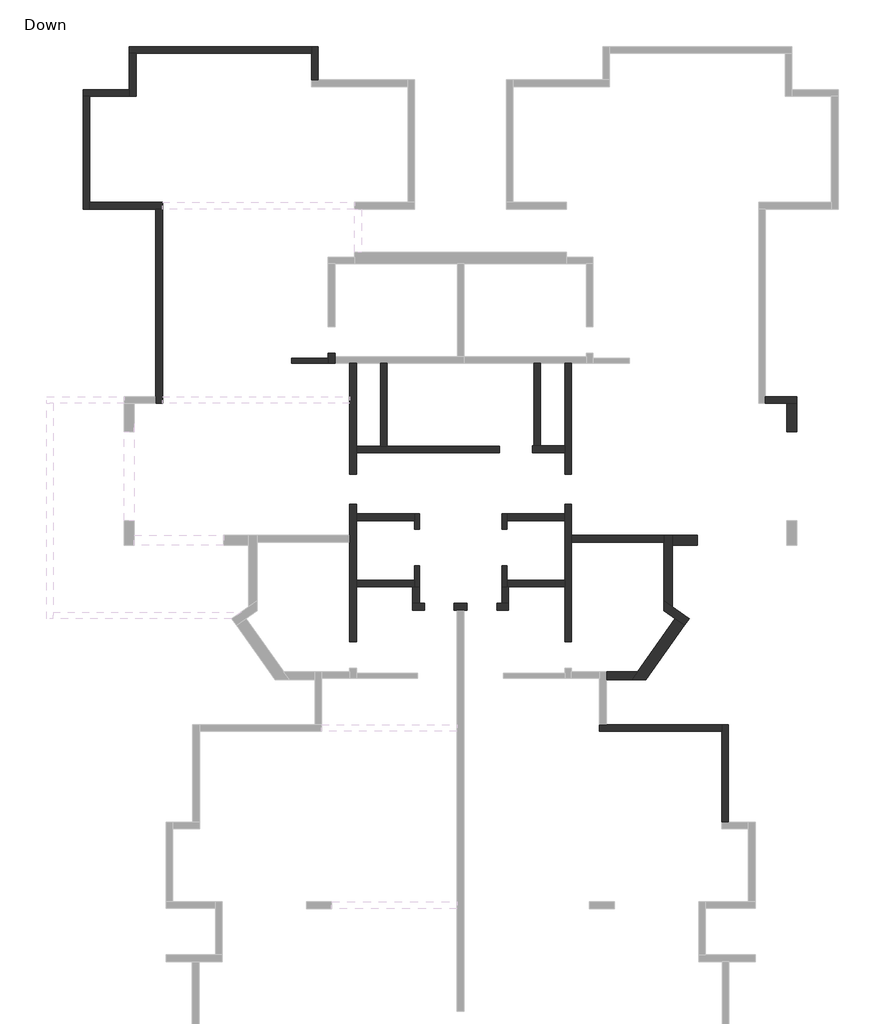
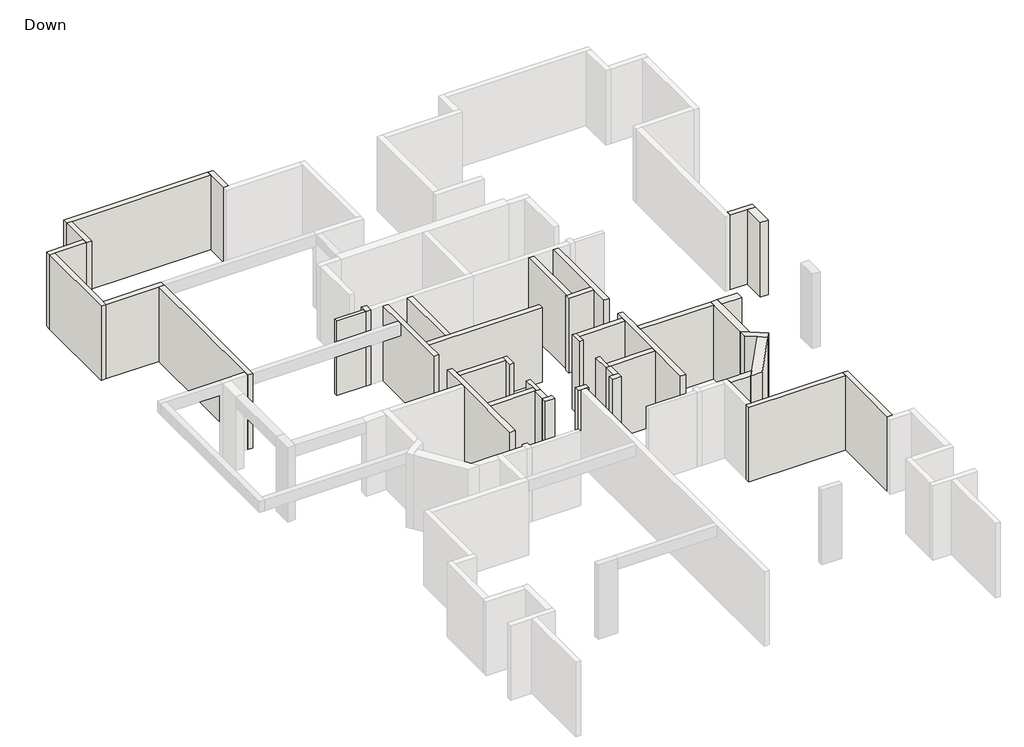
# One storey, part 2 of 3: 40 walls.
"""IFC4 building model written with IfcOpenShell, lengths in millimetres."""

from ifc_helpers import new_model, si_unit, origin, origin_with_axes, place, context, project, spatial, polyline, outline, extrude, faceted_brep, element, save

model = new_model("IFC4")

# Units and contexts
model_context = context("Model", 3, world=origin())
ifc_project = project(units=[si_unit("LENGTHUNIT", "METRE", prefix="MILLI")], contexts=[model_context])

# Site, building, storey
site = spatial("IfcSite", under=ifc_project)
building = spatial("IfcBuilding", under=site)
storey = spatial("IfcBuildingStorey", under=building, Name="Down", Elevation=0.0)

# Walls
placement = place(None, origin())
element("IfcWall", 1, ObjectType="15", at=placement, inside=storey, context=model_context, shape_type="Brep", body=[
    faceted_brep([(27.8998864, 1207.3259107, 0.0), (-1073.0934911, 1207.3259107, 0.0), (-1073.0934911, 1207.3259107, 2800.0), (-1073.0934911, 1207.3259107, 3000.0), (27.8998864, 1207.3259107, 3000.0), (27.8998864, 1207.3259107, 2800.0), (27.8998864, 1057.3259107, 0.0), (27.8998864, 1057.3259107, 3000.0), (-1073.0934911, 1057.3259107, 3000.0), (-1073.0934911, 1057.3259107, 2800.0), (-1073.0934911, 1057.3259107, 0.0)], [[[0, 1, 2, 3, 4, 5]], [[6, 7, 8, 9, 10]], [[1, 0, 6, 10]], [[3, 2, 1, 10, 9, 8]], [[4, 3, 8, 7]], [[0, 5, 4, 7, 6]]]),
])
element("IfcWall", 2, ObjectType="15", at=placement, inside=storey, context=model_context, shape_type="Brep", body=[
    faceted_brep([(2777.2376347, -3950.6211091, 0.0), (2777.2376347, -3491.349586, 0.0), (2777.2376347, -3491.349586, 2800.0), (2777.2376347, -3491.349586, 3000.0), (2777.2376347, -3950.6211091, 3000.0), (2777.2376347, -3950.6211091, 2800.0), (2627.2376347, -3950.6211091, 0.0), (2627.2376347, -3950.6211091, 2800.0), (2627.2376347, -3950.6211091, 3000.0), (2627.2376347, -3691.349586, 3000.0), (2627.2376347, -3491.349586, 3000.0), (2627.2376347, -3491.349586, 0.0), (2627.2376347, -3691.349586, 0.0)], [[[0, 1, 2, 3, 4, 5]], [[6, 7, 8, 9, 10, 11, 12]], [[1, 0, 6, 12, 11]], [[4, 3, 10, 9, 8]], [[0, 5, 4, 8, 7, 6]], [[3, 2, 1, 11, 10]]]),
])
element("IfcWall", 3, ObjectType="15", at=placement, inside=storey, context=model_context, shape_type="Brep", body=[
    faceted_brep([(2777.2376347, -5693.3363409, 0.0), (2777.2376347, -5051.6144866, 0.0), (2777.2376347, -5051.6144866, 2800.0), (2777.2376347, -5051.6144866, 3000.0), (2777.2376347, -5693.3363409, 3000.0), (2627.2376347, -5693.3363409, 0.0), (2627.2376347, -5693.3363409, 3000.0), (2627.2376347, -5493.3363409, 3000.0), (2627.2376347, -5051.6144866, 3000.0), (2627.2376347, -5051.6144866, 2800.0), (2627.2376347, -5051.6144866, 0.0), (2627.2376347, -5493.3363409, 0.0)], [[[0, 1, 2, 3, 4]], [[5, 6, 7, 8, 9, 10, 11]], [[1, 0, 5, 11, 10]], [[3, 2, 1, 10, 9, 8]], [[4, 3, 8, 7, 6]], [[0, 4, 6, 5]]]),
])
element("IfcWall", 4, ObjectType="15", at=placement, inside=storey, context=model_context, shape_type="Brep", body=[
    faceted_brep([(5419.9528665, -3950.6211091, 0.0), (5419.9528665, -3691.349586, 0.0), (5419.9528665, -3491.349586, 0.0), (5419.9528665, -3491.349586, 3000.0), (5419.9528665, -3691.349586, 3000.0), (5419.9528665, -3950.6211091, 3000.0), (5419.9528665, -3950.6211091, 2800.0), (5269.9528665, -3950.6211091, 0.0), (5269.9528665, -3950.6211091, 2800.0), (5269.9528665, -3950.6211091, 3000.0), (5269.9528665, -3491.349586, 3000.0), (5269.9528665, -3491.349586, 2800.0), (5269.9528665, -3491.349586, 0.0)], [[[0, 1, 2, 3, 4, 5, 6]], [[7, 8, 9, 10, 11, 12]], [[2, 1, 0, 7, 12]], [[5, 4, 3, 10, 9]], [[0, 6, 5, 9, 8, 7]], [[3, 2, 12, 11, 10]]]),
])
element("IfcWall", 5, ObjectType="15", at=placement, inside=storey, context=model_context, shape_type="Brep", body=[
    faceted_brep([(5419.9528665, -5693.3363409, 0.0), (5419.9528665, -5493.3363409, 0.0), (5419.9528665, -5051.6144866, 0.0), (5419.9528665, -5051.6144866, 2800.0), (5419.9528665, -5051.6144866, 3000.0), (5419.9528665, -5493.3363409, 3000.0), (5419.9528665, -5693.3363409, 3000.0), (5269.9528665, -5693.3363409, 0.0), (5269.9528665, -5693.3363409, 3000.0), (5269.9528665, -5051.6144866, 3000.0), (5269.9528665, -5051.6144866, 2800.0), (5269.9528665, -5051.6144866, 0.0)], [[[0, 1, 2, 3, 4, 5, 6]], [[7, 8, 9, 10, 11]], [[2, 1, 0, 7, 11]], [[4, 3, 2, 11, 10, 9]], [[6, 5, 4, 9, 8]], [[0, 6, 8, 7]]]),
])
element("IfcWall", 6, ObjectType="20", at=placement, inside=storey, context=model_context, shape_type="Brep", body=[
    faceted_brep([(-275.4113719, 9607.9881624, 0.0), (-275.4113719, 10613.9484273, 0.0), (-275.4113719, 10613.9484273, 3000.0), (-275.4113719, 9607.9881624, 3000.0), (-475.4113719, 9607.9881624, 0.0), (-475.4113719, 9607.9881624, 3000.0), (-475.4113719, 10413.9484273, 3000.0), (-475.4113719, 10613.9484273, 3000.0), (-475.4113719, 10613.9484273, 0.0), (-475.4113719, 10413.9484273, 0.0)], [[[0, 1, 2, 3]], [[4, 5, 6, 7, 8, 9]], [[1, 0, 4, 9, 8]], [[3, 2, 7, 6, 5]], [[0, 3, 5, 4]], [[2, 1, 8, 7]]]),
])
element("IfcWall", 7, ObjectType="20", at=placement, inside=storey, context=model_context, shape_type="Brep", body=[
    faceted_brep([(-475.4113719, 10613.9484273, 0.0), (-5975.4113719, 10613.9484273, 0.0), (-5975.4113719, 10613.9484273, 3000.0), (-475.4113719, 10613.9484273, 3000.0), (-475.4113719, 10413.9484273, 0.0), (-475.4113719, 10413.9484273, 2800.0), (-475.4113719, 10413.9484273, 3000.0), (-5775.4113719, 10413.9484273, 3000.0), (-5975.4113719, 10413.9484273, 3000.0), (-5975.4113719, 10413.9484273, 0.0), (-5775.4113719, 10413.9484273, 0.0)], [[[0, 1, 2, 3]], [[4, 5, 6, 7, 8, 9, 10]], [[1, 0, 4, 10, 9]], [[3, 2, 8, 7, 6]], [[0, 3, 6, 5, 4]], [[2, 1, 9, 8]]]),
])
element("IfcWall", 8, ObjectType="20", at=placement, inside=storey, context=model_context, shape_type="Brep", body=[
    faceted_brep([(-5975.4113719, 10413.9484273, 0.0), (-5975.4113719, 9310.3060432, 0.0), (-5975.4113719, 9110.3060432, 0.0), (-5975.4113719, 9110.3060432, 3000.0), (-5975.4113719, 9310.3060432, 3000.0), (-5975.4113719, 10413.9484273, 3000.0), (-5775.4113719, 10413.9484273, 0.0), (-5775.4113719, 10413.9484273, 2800.0), (-5775.4113719, 10413.9484273, 3000.0), (-5775.4113719, 9110.3060432, 3000.0), (-5775.4113719, 9110.3060432, 2800.0), (-5775.4113719, 9110.3060432, 0.0)], [[[0, 1, 2, 3, 4, 5]], [[6, 7, 8, 9, 10, 11]], [[2, 1, 0, 6, 11]], [[5, 4, 3, 9, 8]], [[0, 5, 8, 7, 6]], [[3, 2, 11, 10, 9]]]),
])
element("IfcWall", 9, ObjectType="20", at=placement, inside=storey, context=model_context, shape_type="Brep", body=[
    faceted_brep([(-5975.4113719, 9310.3060432, 0.0), (-7377.0670011, 9310.3060432, 0.0), (-7377.0670011, 9310.3060432, 3000.0), (-5975.4113719, 9310.3060432, 3000.0), (-5975.4113719, 9110.3060432, 0.0), (-5975.4113719, 9110.3060432, 3000.0), (-7177.0670011, 9110.3060432, 3000.0), (-7377.0670011, 9110.3060432, 3000.0), (-7377.0670011, 9110.3060432, 0.0), (-7177.0670011, 9110.3060432, 0.0)], [[[0, 1, 2, 3]], [[4, 5, 6, 7, 8, 9]], [[1, 0, 4, 9, 8]], [[3, 2, 7, 6, 5]], [[0, 3, 5, 4]], [[2, 1, 8, 7]]]),
])
element("IfcWall", 10, ObjectType="20", at=placement, inside=storey, context=model_context, shape_type="Brep", body=[
    faceted_brep([(-7377.0670011, 9110.3060432, 0.0), (-7377.0670011, 5707.9881624, 0.0), (-7377.0670011, 5707.9881624, 3000.0), (-7377.0670011, 9110.3060432, 3000.0), (-7177.0670011, 9110.3060432, 0.0), (-7177.0670011, 9110.3060432, 2800.0), (-7177.0670011, 9110.3060432, 3000.0), (-7177.0670011, 5907.9881624, 3000.0), (-7177.0670011, 5707.9881624, 3000.0), (-7177.0670011, 5707.9881624, 0.0), (-7177.0670011, 5907.9881624, 0.0)], [[[0, 1, 2, 3]], [[4, 5, 6, 7, 8, 9, 10]], [[1, 0, 4, 10, 9]], [[3, 2, 8, 7, 6]], [[0, 3, 6, 5, 4]], [[2, 1, 9, 8]]]),
])
element("IfcWall", 11, ObjectType="20", at=placement, inside=storey, context=model_context, shape_type="Brep", body=[
    faceted_brep([(-7177.0670011, 5707.9881624, 0.0), (-5177.0670011, 5707.9881624, 0.0), (-4977.0670011, 5707.9881624, 0.0), (-4977.0670011, 5707.9881624, 2550.0), (-4977.0670011, 5707.9881624, 3000.0), (-5177.0670011, 5707.9881624, 3000.0), (-7177.0670011, 5707.9881624, 3000.0), (-7177.0670011, 5907.9881624, 0.0), (-7177.0670011, 5907.9881624, 2800.0), (-7177.0670011, 5907.9881624, 3000.0), (-4977.0670011, 5907.9881624, 3000.0), (-4977.0670011, 5907.9881624, 2550.0), (-4977.0670011, 5907.9881624, 0.0)], [[[0, 1, 2, 3, 4, 5, 6]], [[7, 8, 9, 10, 11, 12]], [[2, 1, 0, 7, 12]], [[6, 5, 4, 10, 9]], [[0, 6, 9, 8, 7]], [[4, 3, 2, 12, 11, 10]]]),
])
element("IfcWall", 12, ObjectType="20", at=placement, inside=storey, context=model_context, shape_type="Brep", body=[
    faceted_brep([(-5177.0670011, 5707.9881624, 0.0), (-5177.0670011, 46.6636591, 0.0), (-5177.0670011, -153.3363409, 0.0), (-5177.0670011, -153.3363409, 3000.0), (-5177.0670011, 46.6636591, 3000.0), (-5177.0670011, 5707.9881624, 3000.0), (-4977.0670011, 5707.9881624, 0.0), (-4977.0670011, 5707.9881624, 2800.0), (-4977.0670011, 5707.9881624, 3000.0), (-4977.0670011, 46.6636591, 3000.0), (-4977.0670011, -153.3363409, 3000.0), (-4977.0670011, -153.3363409, 0.0)], [[[0, 1, 2, 3, 4, 5]], [[6, 7, 8, 9, 10, 11]], [[2, 1, 0, 6, 11]], [[5, 4, 3, 10, 9, 8]], [[0, 5, 8, 7, 6]], [[3, 2, 11, 10]]]),
])
element("IfcWall", 13, ObjectType="20", at=placement, inside=storey, context=model_context, shape_type="Brep", body=[
    faceted_brep([(27.8998864, 1353.021275, 0.0), (27.8998864, 1207.3259107, 0.0), (27.8998864, 1057.3259107, 0.0), (27.8998864, 1057.3259107, 3000.0), (27.8998864, 1207.3259107, 3000.0), (27.8998864, 1353.021275, 3000.0), (27.8998864, 1353.021275, 2800.0), (227.8998864, 1353.021275, 0.0), (227.8998864, 1353.021275, 2800.0), (227.8998864, 1353.021275, 3000.0), (227.8998864, 1257.3259107, 3000.0), (227.8998864, 1057.3259107, 3000.0), (227.8998864, 1057.3259107, 0.0), (227.8998864, 1257.3259107, 0.0)], [[[0, 1, 2, 3, 4, 5, 6]], [[7, 8, 9, 10, 11, 12, 13]], [[2, 1, 0, 7, 13, 12]], [[5, 4, 3, 11, 10, 9]], [[0, 6, 5, 9, 8, 7]], [[3, 2, 12, 11]]]),
])
element("IfcWall", 14, ObjectType="20", at=placement, inside=storey, context=model_context, shape_type="Brep", body=[
    faceted_brep([(675.9131314, 1057.3259107, 0.0), (675.9131314, -2295.9853475, 0.0), (675.9131314, -2295.9853475, 2800.0), (675.9131314, -2295.9853475, 3000.0), (675.9131314, -153.3363409, 3000.0), (675.9131314, 46.6636591, 3000.0), (675.9131314, 1057.3259107, 3000.0), (675.9131314, 1057.3259107, 2800.0), (875.9131314, 1057.3259107, 0.0), (875.9131314, 1057.3259107, 3000.0), (875.9131314, -1441.6807118, 3000.0), (875.9131314, -1641.6807118, 3000.0), (875.9131314, -2295.9853475, 3000.0), (875.9131314, -2295.9853475, 2800.0), (875.9131314, -2295.9853475, 0.0), (875.9131314, -1641.6807118, 0.0), (875.9131314, -1441.6807118, 0.0)], [[[0, 1, 2, 3, 4, 5, 6, 7]], [[8, 9, 10, 11, 12, 13, 14, 15, 16]], [[1, 0, 8, 16, 15, 14]], [[3, 2, 1, 14, 13, 12]], [[6, 5, 4, 3, 12, 11, 10, 9]], [[0, 7, 6, 9, 8]]]),
])
element("IfcWall", 15, ObjectType="20", at=placement, inside=storey, context=model_context, shape_type="Brep", body=[
    faceted_brep([(875.9131314, -1641.6807118, 0.0), (5199.4230652, -1641.6807118, 0.0), (5199.4230652, -1641.6807118, 2800.0), (5199.4230652, -1641.6807118, 3000.0), (875.9131314, -1641.6807118, 3000.0), (875.9131314, -1641.6807118, 2800.0), (875.9131314, -1441.6807118, 0.0), (875.9131314, -1441.6807118, 3000.0), (1608.3634625, -1441.6807118, 3000.0), (1808.3634625, -1441.6807118, 3000.0), (5199.4230652, -1441.6807118, 3000.0), (5199.4230652, -1441.6807118, 2800.0), (5199.4230652, -1441.6807118, 0.0), (1808.3634625, -1441.6807118, 0.0), (1608.3634625, -1441.6807118, 0.0)], [[[0, 1, 2, 3, 4, 5]], [[6, 7, 8, 9, 10, 11, 12, 13, 14]], [[1, 0, 6, 14, 13, 12]], [[3, 2, 1, 12, 11, 10]], [[4, 3, 10, 9, 8, 7]], [[0, 5, 4, 7, 6]]]),
])
element("IfcWall", 16, ObjectType="20", at=placement, inside=storey, context=model_context, shape_type="SweptSolid", body=[
    extrude(outline(polyline([(1808.3634625, 1057.3259107), (1808.3634625, -1441.6807118), (1608.3634625, -1441.6807118), (1608.3634625, 1057.3259107), (1808.3634625, 1057.3259107)])), origin_with_axes(), (0.0, 0.0, 1.0), 3000.0),
])
element("IfcWall", 17, ObjectType="20", at=placement, inside=storey, context=model_context, shape_type="Brep", body=[
    faceted_brep([(675.9131314, -3195.6542217, 0.0), (675.9131314, -4140.6873343, 0.0), (675.9131314, -4340.6873343, 0.0), (675.9131314, -7341.6807118, 0.0), (675.9131314, -7341.6807118, 2800.0), (675.9131314, -7341.6807118, 3000.0), (675.9131314, -4340.6873343, 3000.0), (675.9131314, -4140.6873343, 3000.0), (675.9131314, -3195.6542217, 3000.0), (675.9131314, -3195.6542217, 2800.0), (875.9131314, -3195.6542217, 0.0), (875.9131314, -3195.6542217, 2800.0), (875.9131314, -3195.6542217, 3000.0), (875.9131314, -3491.349586, 3000.0), (875.9131314, -3691.349586, 3000.0), (875.9131314, -5493.3363409, 3000.0), (875.9131314, -5693.3363409, 3000.0), (875.9131314, -7341.6807118, 3000.0), (875.9131314, -7341.6807118, 2800.0), (875.9131314, -7341.6807118, 0.0), (875.9131314, -5693.3363409, 0.0), (875.9131314, -5493.3363409, 0.0), (875.9131314, -3691.349586, 0.0), (875.9131314, -3491.349586, 0.0)], [[[0, 1, 2, 3, 4, 5, 6, 7, 8, 9]], [[10, 11, 12, 13, 14, 15, 16, 17, 18, 19, 20, 21, 22, 23]], [[3, 2, 1, 0, 10, 23, 22, 21, 20, 19]], [[5, 4, 3, 19, 18, 17]], [[8, 7, 6, 5, 17, 16, 15, 14, 13, 12]], [[0, 9, 8, 12, 11, 10]]]),
])
element("IfcWall", 18, ObjectType="20", at=placement, inside=storey, context=model_context, shape_type="Brep", body=[
    faceted_brep([(875.9131314, -5693.3363409, 0.0), (2577.2376347, -5693.3363409, 0.0), (2627.2376347, -5693.3363409, 0.0), (2627.2376347, -5693.3363409, 3000.0), (2577.2376347, -5693.3363409, 3000.0), (875.9131314, -5693.3363409, 3000.0), (875.9131314, -5693.3363409, 2800.0), (875.9131314, -5493.3363409, 0.0), (875.9131314, -5493.3363409, 3000.0), (2627.2376347, -5493.3363409, 3000.0), (2627.2376347, -5493.3363409, 0.0)], [[[0, 1, 2, 3, 4, 5, 6]], [[7, 8, 9, 10]], [[2, 1, 0, 7, 10]], [[5, 4, 3, 9, 8]], [[0, 6, 5, 8, 7]], [[3, 2, 10, 9]]]),
])
element("IfcWall", 19, ObjectType="20", at=placement, inside=storey, context=model_context, shape_type="Brep", body=[
    faceted_brep([(2627.2376347, -3491.349586, 0.0), (875.9131314, -3491.349586, 0.0), (875.9131314, -3491.349586, 2800.0), (875.9131314, -3491.349586, 3000.0), (2627.2376347, -3491.349586, 3000.0), (2627.2376347, -3691.349586, 0.0), (2627.2376347, -3691.349586, 3000.0), (875.9131314, -3691.349586, 3000.0), (875.9131314, -3691.349586, 0.0)], [[[0, 1, 2, 3, 4]], [[5, 6, 7, 8]], [[1, 0, 5, 8]], [[4, 3, 7, 6]], [[0, 4, 6, 5]], [[3, 2, 1, 8, 7]]]),
])
element("IfcWall", 20, ObjectType="20", at=placement, inside=storey, context=model_context, shape_type="Brep", body=[
    faceted_brep([(2577.2376347, -5693.3363409, 0.0), (2577.2376347, -6191.6807118, 0.0), (2577.2376347, -6191.6807118, 3000.0), (2577.2376347, -5693.3363409, 3000.0), (2577.2376347, -5693.3363409, 2800.0), (2777.2376347, -5693.3363409, 0.0), (2777.2376347, -5693.3363409, 3000.0), (2777.2376347, -6191.6807118, 3000.0), (2777.2376347, -6191.6807118, 2800.0), (2777.2376347, -6191.6807118, 0.0), (2627.2376347, -5693.3363409, 0.0), (2627.2376347, -5693.3363409, 3000.0)], [[[0, 1, 2, 3, 4]], [[5, 6, 7, 8, 9]], [[1, 0, 10, 5, 9]], [[3, 2, 7, 6, 11]], [[0, 4, 3, 11, 6, 5, 10]], [[2, 1, 9, 8, 7]]]),
])
element("IfcWall", 21, ObjectType="20", at=placement, inside=storey, context=model_context, shape_type="Brep", body=[
    faceted_brep([(2577.2376347, -6391.6807118, 0.0), (2928.2310122, -6391.6807118, 0.0), (2928.2310122, -6391.6807118, 2800.0), (2928.2310122, -6391.6807118, 3000.0), (2577.2376347, -6391.6807118, 3000.0), (2577.2376347, -6391.6807118, 2800.0), (2577.2376347, -6191.6807118, 0.0), (2577.2376347, -6191.6807118, 3000.0), (2777.2376347, -6191.6807118, 3000.0), (2928.2310122, -6191.6807118, 3000.0), (2928.2310122, -6191.6807118, 2800.0), (2928.2310122, -6191.6807118, 0.0), (2777.2376347, -6191.6807118, 0.0)], [[[0, 1, 2, 3, 4, 5]], [[6, 7, 8, 9, 10, 11, 12]], [[1, 0, 6, 12, 11]], [[3, 2, 1, 11, 10, 9]], [[4, 3, 9, 8, 7]], [[0, 5, 4, 7, 6]]]),
])
element("IfcWall", 22, ObjectType="20", at=placement, inside=storey, context=model_context, shape_type="Brep", body=[
    faceted_brep([(3827.8998864, -6391.6807118, 0.0), (3923.5952506, -6391.6807118, 0.0), (4123.5952506, -6391.6807118, 0.0), (4224.2575022, -6391.6807118, 0.0), (4224.2575022, -6391.6807118, 2800.0), (4224.2575022, -6391.6807118, 3000.0), (4123.5952506, -6391.6807118, 3000.0), (3923.5952506, -6391.6807118, 3000.0), (3827.8998864, -6391.6807118, 3000.0), (3827.8998864, -6391.6807118, 2800.0), (3827.8998864, -6191.6807118, 0.0), (3827.8998864, -6191.6807118, 2800.0), (3827.8998864, -6191.6807118, 3000.0), (4224.2575022, -6191.6807118, 3000.0), (4224.2575022, -6191.6807118, 2800.0), (4224.2575022, -6191.6807118, 0.0)], [[[0, 1, 2, 3, 4, 5, 6, 7, 8, 9]], [[10, 11, 12, 13, 14, 15]], [[3, 2, 1, 0, 10, 15]], [[5, 4, 3, 15, 14, 13]], [[8, 7, 6, 5, 13, 12]], [[0, 9, 8, 12, 11, 10]]]),
])
element("IfcWall", 23, ObjectType="20", at=placement, inside=storey, context=model_context, shape_type="Brep", body=[
    faceted_brep([(13224.2575022, -153.3363409, 0.0), (13875.1499872, -153.3363409, 0.0), (14175.1499872, -153.3363409, 0.0), (14175.1499872, -153.3363409, 2550.0), (14175.1499872, -153.3363409, 3000.0), (13875.1499872, -153.3363409, 3000.0), (13224.2575022, -153.3363409, 3000.0), (13224.2575022, 46.6636591, 0.0), (13224.2575022, 46.6636591, 3000.0), (14175.1499872, 46.6636591, 3000.0), (14175.1499872, 46.6636591, 2550.0), (14175.1499872, 46.6636591, 0.0)], [[[0, 1, 2, 3, 4, 5, 6]], [[7, 8, 9, 10, 11]], [[2, 1, 0, 7, 11]], [[6, 5, 4, 9, 8]], [[0, 6, 8, 7]], [[4, 3, 2, 11, 10, 9]]]),
])
element("IfcWall", 24, ObjectType="20", at=placement, inside=storey, context=model_context, shape_type="Brep", body=[
    faceted_brep([(7169.9528665, 1057.3259107, 0.0), (7169.9528665, -1440.3562085, 0.0), (7169.9528665, -1640.3562085, 0.0), (7169.9528665, -2295.9853475, 0.0), (7169.9528665, -2295.9853475, 2800.0), (7169.9528665, -2295.9853475, 3000.0), (7169.9528665, -1640.3562085, 3000.0), (7169.9528665, -1440.3562085, 3000.0), (7169.9528665, 1057.3259107, 3000.0), (7369.9528665, 1057.3259107, 0.0), (7369.9528665, 1057.3259107, 2800.0), (7369.9528665, 1057.3259107, 3000.0), (7369.9528665, 46.6636591, 3000.0), (7369.9528665, -153.3363409, 3000.0), (7369.9528665, -2295.9853475, 3000.0), (7369.9528665, -2295.9853475, 2800.0), (7369.9528665, -2295.9853475, 0.0)], [[[0, 1, 2, 3, 4, 5, 6, 7, 8]], [[9, 10, 11, 12, 13, 14, 15, 16]], [[3, 2, 1, 0, 9, 16]], [[5, 4, 3, 16, 15, 14]], [[8, 7, 6, 5, 14, 13, 12, 11]], [[0, 8, 11, 10, 9]]]),
])
element("IfcWall", 25, ObjectType="20", at=placement, inside=storey, context=model_context, shape_type="SweptSolid", body=[
    extrude(outline(polyline([(6438.8270387, 1057.3259107), (6438.8270387, -1440.3562085), (6238.8270387, -1440.3562085), (6238.8270387, 1057.3259107), (6438.8270387, 1057.3259107)])), origin_with_axes(), (0.0, 0.0, 1.0), 3000.0),
])
element("IfcWall", 26, ObjectType="20", at=placement, inside=storey, context=model_context, shape_type="Brep", body=[
    faceted_brep([(7169.9528665, -3195.6542217, 0.0), (7169.9528665, -3491.349586, 0.0), (7169.9528665, -3691.349586, 0.0), (7169.9528665, -5493.3363409, 0.0), (7169.9528665, -5693.3363409, 0.0), (7169.9528665, -7341.6807118, 0.0), (7169.9528665, -7341.6807118, 2800.0), (7169.9528665, -7341.6807118, 3000.0), (7169.9528665, -5693.3363409, 3000.0), (7169.9528665, -5493.3363409, 3000.0), (7169.9528665, -3691.349586, 3000.0), (7169.9528665, -3491.349586, 3000.0), (7169.9528665, -3195.6542217, 3000.0), (7169.9528665, -3195.6542217, 2800.0), (7369.9528665, -3195.6542217, 0.0), (7369.9528665, -3195.6542217, 2800.0), (7369.9528665, -3195.6542217, 3000.0), (7369.9528665, -4140.6873343, 3000.0), (7369.9528665, -4340.6873343, 3000.0), (7369.9528665, -7341.6807118, 3000.0), (7369.9528665, -7341.6807118, 2800.0), (7369.9528665, -7341.6807118, 0.0), (7369.9528665, -4340.6873343, 0.0), (7369.9528665, -4140.6873343, 0.0)], [[[0, 1, 2, 3, 4, 5, 6, 7, 8, 9, 10, 11, 12, 13]], [[14, 15, 16, 17, 18, 19, 20, 21, 22, 23]], [[5, 4, 3, 2, 1, 0, 14, 23, 22, 21]], [[7, 6, 5, 21, 20, 19]], [[12, 11, 10, 9, 8, 7, 19, 18, 17, 16]], [[0, 13, 12, 16, 15, 14]]]),
])
element("IfcWall", 27, ObjectType="20", at=placement, inside=storey, context=model_context, shape_type="Brep", body=[
    faceted_brep([(7169.9528665, -5493.3363409, 0.0), (5419.9528665, -5493.3363409, 0.0), (5419.9528665, -5493.3363409, 3000.0), (7169.9528665, -5493.3363409, 3000.0), (7169.9528665, -5693.3363409, 0.0), (7169.9528665, -5693.3363409, 2800.0), (7169.9528665, -5693.3363409, 3000.0), (5469.9528665, -5693.3363409, 3000.0), (5419.9528665, -5693.3363409, 3000.0), (5419.9528665, -5693.3363409, 0.0), (5469.9528665, -5693.3363409, 0.0)], [[[0, 1, 2, 3]], [[4, 5, 6, 7, 8, 9, 10]], [[1, 0, 4, 10, 9]], [[3, 2, 8, 7, 6]], [[0, 3, 6, 5, 4]], [[2, 1, 9, 8]]]),
])
element("IfcWall", 28, ObjectType="20", at=placement, inside=storey, context=model_context, shape_type="Brep", body=[
    faceted_brep([(5419.9528665, -3691.349586, 0.0), (7169.9528665, -3691.349586, 0.0), (7169.9528665, -3691.349586, 3000.0), (5419.9528665, -3691.349586, 3000.0), (5419.9528665, -3491.349586, 0.0), (5419.9528665, -3491.349586, 3000.0), (7169.9528665, -3491.349586, 3000.0), (7169.9528665, -3491.349586, 2800.0), (7169.9528665, -3491.349586, 0.0)], [[[0, 1, 2, 3]], [[4, 5, 6, 7, 8]], [[1, 0, 4, 8]], [[3, 2, 6, 5]], [[0, 3, 5, 4]], [[2, 1, 8, 7, 6]]]),
])
element("IfcWall", 29, ObjectType="20", at=placement, inside=storey, context=model_context, shape_type="Brep", body=[
    faceted_brep([(5269.9528665, -5693.3363409, 0.0), (5269.9528665, -6191.6807118, 0.0), (5269.9528665, -6191.6807118, 2800.0), (5269.9528665, -6191.6807118, 3000.0), (5269.9528665, -5693.3363409, 3000.0), (5469.9528665, -5693.3363409, 0.0), (5469.9528665, -5693.3363409, 2800.0), (5469.9528665, -5693.3363409, 3000.0), (5469.9528665, -6191.6807118, 3000.0), (5469.9528665, -6191.6807118, 0.0), (5419.9528665, -5693.3363409, 0.0), (5419.9528665, -5693.3363409, 3000.0)], [[[0, 1, 2, 3, 4]], [[5, 6, 7, 8, 9]], [[1, 0, 10, 5, 9]], [[4, 3, 8, 7, 11]], [[0, 4, 11, 7, 6, 5, 10]], [[3, 2, 1, 9, 8]]]),
])
element("IfcWall", 30, ObjectType="20", at=placement, inside=storey, context=model_context, shape_type="Brep", body=[
    faceted_brep([(5469.9528665, -6191.6807118, 0.0), (5269.9528665, -6191.6807118, 0.0), (5118.959489, -6191.6807118, 0.0), (5118.959489, -6191.6807118, 2800.0), (5118.959489, -6191.6807118, 3000.0), (5269.9528665, -6191.6807118, 3000.0), (5469.9528665, -6191.6807118, 3000.0), (5469.9528665, -6391.6807118, 0.0), (5469.9528665, -6391.6807118, 2800.0), (5469.9528665, -6391.6807118, 3000.0), (5118.959489, -6391.6807118, 3000.0), (5118.959489, -6391.6807118, 2800.0), (5118.959489, -6391.6807118, 0.0)], [[[0, 1, 2, 3, 4, 5, 6]], [[7, 8, 9, 10, 11, 12]], [[2, 1, 0, 7, 12]], [[4, 3, 2, 12, 11, 10]], [[6, 5, 4, 10, 9]], [[0, 6, 9, 8, 7]]]),
])
element("IfcWall", 31, ObjectType="20", at=placement, inside=storey, context=model_context, shape_type="Brep", body=[
    faceted_brep([(12107.370085, -12796.3164734, 0.0), (12107.370085, -9845.6542217, 0.0), (12107.370085, -9845.6542217, 3000.0), (12107.370085, -12796.3164734, 3000.0), (11907.370085, -12796.3164734, 0.0), (11907.370085, -12796.3164734, 3000.0), (11907.370085, -10045.6542217, 3000.0), (11907.370085, -9845.6542217, 3000.0), (11907.370085, -9845.6542217, 0.0), (11907.370085, -10045.6542217, 0.0)], [[[0, 1, 2, 3]], [[4, 5, 6, 7, 8, 9]], [[1, 0, 4, 9, 8]], [[3, 2, 7, 6, 5]], [[0, 3, 5, 4]], [[2, 1, 8, 7]]]),
])
element("IfcWall", 32, ObjectType="20", at=placement, inside=storey, context=model_context, shape_type="Brep", body=[
    faceted_brep([(11907.370085, -9845.6542217, 0.0), (8420.6151181, -9845.6542217, 0.0), (8220.6151181, -9845.6542217, 0.0), (8220.6151181, -9845.6542217, 2550.0), (8220.6151181, -9845.6542217, 3000.0), (8420.6151181, -9845.6542217, 3000.0), (11907.370085, -9845.6542217, 3000.0), (11907.370085, -10045.6542217, 0.0), (11907.370085, -10045.6542217, 2800.0), (11907.370085, -10045.6542217, 3000.0), (8220.6151181, -10045.6542217, 3000.0), (8220.6151181, -10045.6542217, 2550.0), (8220.6151181, -10045.6542217, 0.0)], [[[0, 1, 2, 3, 4, 5, 6]], [[7, 8, 9, 10, 11, 12]], [[2, 1, 0, 7, 12]], [[6, 5, 4, 10, 9]], [[0, 6, 9, 8, 7]], [[4, 3, 2, 12, 11, 10]]]),
])
element("IfcWall", 33, ObjectType="20", at=placement, inside=storey, context=model_context, shape_type="Brep", body=[
    faceted_brep([(10167.9817051, -4140.6873343, 0.0), (7369.9528665, -4140.6873343, 0.0), (7369.9528665, -4140.6873343, 2800.0), (7369.9528665, -4140.6873343, 3000.0), (10167.9817051, -4140.6873343, 3000.0), (10167.9817051, -4340.6873343, 0.0), (10167.9817051, -4340.6873343, 2800.0), (10167.9817051, -4340.6873343, 3000.0), (7369.9528665, -4340.6873343, 3000.0), (7369.9528665, -4340.6873343, 2800.0), (7369.9528665, -4340.6873343, 0.0)], [[[0, 1, 2, 3, 4]], [[5, 6, 7, 8, 9, 10]], [[1, 0, 5, 10]], [[4, 3, 8, 7]], [[0, 4, 7, 6, 5]], [[3, 2, 1, 10, 9, 8]]]),
])
element("IfcWall", 34, ObjectType="20", at=placement, inside=storey, context=model_context, shape_type="Brep", body=[
    faceted_brep([(6199.754191, -1640.3562085, 0.0), (7169.9528665, -1640.3562085, 0.0), (7169.9528665, -1640.3562085, 2800.0), (7169.9528665, -1640.3562085, 3000.0), (6199.754191, -1640.3562085, 3000.0), (6199.754191, -1640.3562085, 2800.0), (6199.754191, -1440.3562085, 0.0), (6199.754191, -1440.3562085, 3000.0), (6238.8270387, -1440.3562085, 3000.0), (6438.8270387, -1440.3562085, 3000.0), (7169.9528665, -1440.3562085, 3000.0), (7169.9528665, -1440.3562085, 0.0), (6438.8270387, -1440.3562085, 0.0), (6238.8270387, -1440.3562085, 0.0), (6199.754191, -1441.6807118, 3000.0)], [[[0, 1, 2, 3, 4, 5]], [[6, 7, 8, 9, 10, 11, 12, 13]], [[1, 0, 6, 13, 12, 11]], [[4, 3, 10, 9, 8, 7, 14]], [[0, 5, 4, 14, 7, 6]], [[3, 2, 1, 11, 10]]]),
])
element("IfcWall", 35, ObjectType="25", at=placement, inside=storey, context=model_context, shape_type="Brep", body=[
    faceted_brep([(8420.6151181, -8497.6409767, 0.0), (9191.6671278, -8497.6409767, 0.0), (9191.6671278, -8497.6409767, 3000.0), (8420.6151181, -8497.6409767, 3000.0), (8420.6151181, -8247.6409767, 0.0), (8420.6151181, -8247.6409767, 3000.0), (9369.2987068, -8247.6409767, 3000.0), (9369.2987068, -8247.6409767, 2800.0), (9369.2987068, -8247.6409767, 0.0)], [[[0, 1, 2, 3]], [[4, 5, 6, 7, 8]], [[1, 0, 4, 8]], [[3, 2, 6, 5]], [[0, 3, 5, 4]], [[2, 1, 8, 7, 6]]]),
])
element("IfcWall", 36, ObjectType="25", at=placement, inside=storey, context=model_context, shape_type="Brep", body=[
    faceted_brep([(10931.7636873, -6652.8905163, 0.0), (10417.9817051, -6287.3148751, 0.0), (10167.9817051, -6109.4302597, 0.0), (10167.9817051, -6109.4302597, 3000.0), (10417.9817051, -6287.3148751, 3000.0), (10931.7636873, -6652.8905163, 3000.0), (10786.9618715, -6856.6856644, 0.0), (10786.9618715, -6856.6856644, 3000.0), (10501.7850127, -6653.7713609, 3000.0), (10167.9817051, -6416.257469, 3000.0), (10167.9817051, -6416.257469, 2800.0), (10167.9817051, -6416.257469, 0.0), (10501.7850127, -6653.7713609, 0.0)], [[[0, 1, 2, 3, 4, 5]], [[6, 7, 8, 9, 10, 11, 12]], [[2, 1, 0, 6, 12, 11]], [[5, 4, 3, 9, 8, 7]], [[0, 5, 7, 6]], [[3, 2, 11, 10, 9]]]),
])
element("IfcWall", 37, ObjectType="25", at=placement, inside=storey, context=model_context, shape_type="Brep", body=[
    faceted_brep([(10417.9817051, -6287.3148751, 0.0), (10417.9817051, -4440.6873343, 0.0), (10417.9817051, -4140.6873343, 0.0), (10417.9817051, -4140.6873343, 3000.0), (10417.9817051, -4440.6873343, 3000.0), (10417.9817051, -6287.3148751, 3000.0), (10167.9817051, -6109.4302597, 0.0), (10167.9817051, -6109.4302597, 3000.0), (10167.9817051, -4340.6873343, 3000.0), (10167.9817051, -4140.6873343, 3000.0), (10167.9817051, -4140.6873343, 0.0), (10167.9817051, -4340.6873343, 0.0)], [[[0, 1, 2, 3, 4, 5]], [[6, 7, 8, 9, 10, 11]], [[2, 1, 0, 6, 11, 10]], [[5, 4, 3, 9, 8, 7]], [[0, 5, 7, 6]], [[3, 2, 10, 9]]]),
])
element("IfcWall", 38, ObjectType="30", at=placement, inside=storey, context=model_context, shape_type="Brep", body=[
    faceted_brep([(13875.1499872, -153.3363409, 0.0), (13875.1499872, -1013.3363409, 0.0), (13875.1499872, -1013.3363409, 2550.0), (13875.1499872, -1013.3363409, 2800.0), (13875.1499872, -1013.3363409, 3000.0), (13875.1499872, -153.3363409, 3000.0), (13875.1499872, -153.3363409, 2800.0), (14175.1499872, -153.3363409, 0.0), (14175.1499872, -153.3363409, 2800.0), (14175.1499872, -153.3363409, 3000.0), (14175.1499872, -1013.3363409, 3000.0), (14175.1499872, -1013.3363409, 2800.0), (14175.1499872, -1013.3363409, 0.0), (14174.4026477, -1013.3363409, 3000.0)], [[[0, 1, 2, 3, 4, 5, 6]], [[7, 8, 9, 10, 11, 12]], [[1, 0, 7, 12]], [[4, 3, 2, 1, 12, 11, 10, 13]], [[5, 4, 13, 10, 9]], [[0, 6, 5, 9, 8, 7]]]),
])
element("IfcWall", 39, ObjectType="30", at=placement, inside=storey, context=model_context, shape_type="Brep", body=[
    faceted_brep([(10417.9817051, -4440.6873343, 0.0), (11177.9817051, -4440.6873343, 0.0), (11177.9817051, -4440.6873343, 2550.0), (11177.9817051, -4440.6873343, 3000.0), (10417.9817051, -4440.6873343, 3000.0), (10417.9817051, -4440.6873343, 2800.0), (10417.9817051, -4140.6873343, 0.0), (10417.9817051, -4140.6873343, 3000.0), (11177.9817051, -4140.6873343, 3000.0), (11177.9817051, -4140.6873343, 2550.0), (11177.9817051, -4140.6873343, 0.0)], [[[0, 1, 2, 3, 4, 5]], [[6, 7, 8, 9, 10]], [[1, 0, 6, 10]], [[3, 2, 1, 10, 9, 8]], [[4, 3, 8, 7]], [[0, 5, 4, 7, 6]]]),
])
element("IfcWall", 40, ObjectType="35", at=placement, inside=storey, context=model_context, shape_type="Brep", body=[
    faceted_brep([(9621.0199391, -8497.6409767, 0.0), (10786.9618715, -6856.6856644, 0.0), (10786.9618715, -6856.6856644, 3000.0), (9621.0199391, -8497.6409767, 3000.0), (9191.6671278, -8497.6409767, 0.0), (9191.6671278, -8497.6409767, 3000.0), (9369.2987068, -8247.6409767, 3000.0), (10501.7850127, -6653.7713609, 3000.0), (10501.7850127, -6653.7713609, 2800.0), (10501.7850127, -6653.7713609, 0.0), (9369.2987068, -8247.6409767, 0.0)], [[[0, 1, 2, 3]], [[4, 5, 6, 7, 8, 9, 10]], [[1, 0, 4, 10, 9]], [[3, 2, 7, 6, 5]], [[2, 1, 9, 8, 7]], [[0, 3, 5, 4]]]),
])

save(model, "model.ifc")

# Revit data of these elements
# Type "15"
#   Layers, outside or top first: 15 cm "Concrete" (function 1)
# Type "20"
#   Layers, outside or top first: 20 cm "Concrete" (function 1)
# Type "25"
#   Layers, outside or top first: 25 cm "Concrete" (function 1)
# Type "30"
#   Layers, outside or top first: 30 cm "Concrete" (function 1)
# Type "35"
#   Layers, outside or top first: 35 cm "Concrete" (function 1)
# Element 1 (IfcWall, "15")
#   Comments = ""
#   Mark = "W90"
#   SOFiSTiK_AMG_Comments = ""
#   Top Offset = 0 cm
#   Base Offset = 0 cm
#   wall height = 300 cm
#   SOFiSTiK_AMG_Scheduled = yes
#   SOFiSTiK_AMG_Adjusted = yes
#   Phase Created = New Construction
#   Base Constraint = Down
#   Top Constraint = Typical Floor
#   Materials on its faces: "Concrete"
# Element 2 (IfcWall, "15")
#   Comments = ""
#   Mark = "W91"
#   SOFiSTiK_AMG_Comments = ""
#   Top Offset = 0 cm
#   Base Offset = 0 cm
#   wall height = 300 cm
#   SOFiSTiK_AMG_Scheduled = yes
#   SOFiSTiK_AMG_Adjusted = yes
#   Phase Created = New Construction
#   Base Constraint = Down
#   Top Constraint = Typical Floor
#   Materials on its faces: "Concrete"
# Element 3 (IfcWall, "15")
#   Comments = ""
#   Mark = "W92"
#   SOFiSTiK_AMG_Comments = ""
#   Top Offset = 0 cm
#   Base Offset = 0 cm
#   wall height = 300 cm
#   SOFiSTiK_AMG_Scheduled = yes
#   SOFiSTiK_AMG_Adjusted = yes
#   Phase Created = New Construction
#   Base Constraint = Down
#   Top Constraint = Typical Floor
#   Materials on its faces: "Concrete"
# Element 4 (IfcWall, "15")
#   Comments = ""
#   Mark = "W95"
#   SOFiSTiK_AMG_Comments = ""
#   Top Offset = 0 cm
#   Base Offset = 0 cm
#   wall height = 300 cm
#   SOFiSTiK_AMG_Scheduled = yes
#   SOFiSTiK_AMG_Adjusted = yes
#   Phase Created = New Construction
#   Base Constraint = Down
#   Top Constraint = Typical Floor
#   Materials on its faces: "Concrete"
# Element 5 (IfcWall, "15")
#   Comments = ""
#   Mark = "W96"
#   SOFiSTiK_AMG_Comments = ""
#   Top Offset = 0 cm
#   Base Offset = 0 cm
#   wall height = 300 cm
#   SOFiSTiK_AMG_Scheduled = yes
#   SOFiSTiK_AMG_Adjusted = yes
#   Phase Created = New Construction
#   Base Constraint = Down
#   Top Constraint = Typical Floor
#   Materials on its faces: "Concrete"
# Element 6 (IfcWall, "20")
#   Comments = ""
#   Mark = "W4"
#   SOFiSTiK_AMG_Comments = ""
#   Top Offset = 0 cm
#   Base Offset = 0 cm
#   wall height = 300 cm
#   SOFiSTiK_AMG_Scheduled = yes
#   SOFiSTiK_AMG_Adjusted = yes
#   Phase Created = New Construction
#   Base Constraint = Down
#   Top Constraint = Typical Floor
#   Materials on its faces: "Concrete"
# Element 7 (IfcWall, "20")
#   Comments = ""
#   Mark = "W5"
#   SOFiSTiK_AMG_Comments = ""
#   Top Offset = 0 cm
#   Base Offset = 0 cm
#   wall height = 300 cm
#   SOFiSTiK_AMG_Scheduled = yes
#   SOFiSTiK_AMG_Adjusted = yes
#   Phase Created = New Construction
#   Base Constraint = Down
#   Top Constraint = Typical Floor
#   Materials on its faces: "Concrete"
# Element 8 (IfcWall, "20")
#   Comments = ""
#   Mark = "W6"
#   SOFiSTiK_AMG_Comments = ""
#   Top Offset = 0 cm
#   Base Offset = 0 cm
#   wall height = 300 cm
#   SOFiSTiK_AMG_Scheduled = yes
#   SOFiSTiK_AMG_Adjusted = yes
#   Phase Created = New Construction
#   Base Constraint = Down
#   Top Constraint = Typical Floor
#   Materials on its faces: "Concrete"
# Element 9 (IfcWall, "20")
#   Comments = ""
#   Mark = "W7"
#   SOFiSTiK_AMG_Comments = ""
#   Top Offset = 0 cm
#   Base Offset = 0 cm
#   wall height = 300 cm
#   SOFiSTiK_AMG_Scheduled = yes
#   SOFiSTiK_AMG_Adjusted = yes
#   Phase Created = New Construction
#   Base Constraint = Down
#   Top Constraint = Typical Floor
#   Materials on its faces: "Concrete"
# Element 10 (IfcWall, "20")
#   Comments = ""
#   Mark = "W8"
#   SOFiSTiK_AMG_Comments = ""
#   Top Offset = 0 cm
#   Base Offset = 0 cm
#   wall height = 300 cm
#   SOFiSTiK_AMG_Scheduled = yes
#   SOFiSTiK_AMG_Adjusted = yes
#   Phase Created = New Construction
#   Base Constraint = Down
#   Top Constraint = Typical Floor
#   Materials on its faces: "Concrete"
# Element 11 (IfcWall, "20")
#   Comments = ""
#   Mark = "W9"
#   SOFiSTiK_AMG_Comments = ""
#   Top Offset = 0 cm
#   Base Offset = 0 cm
#   wall height = 300 cm
#   SOFiSTiK_AMG_Scheduled = yes
#   SOFiSTiK_AMG_Adjusted = yes
#   Phase Created = New Construction
#   Base Constraint = Down
#   Top Constraint = Typical Floor
#   Materials on its faces: "Concrete"
# Element 12 (IfcWall, "20")
#   Comments = ""
#   Mark = "W10"
#   SOFiSTiK_AMG_Comments = ""
#   Top Offset = 0 cm
#   Base Offset = 0 cm
#   wall height = 300 cm
#   SOFiSTiK_AMG_Scheduled = yes
#   SOFiSTiK_AMG_Adjusted = yes
#   Phase Created = New Construction
#   Base Constraint = Down
#   Top Constraint = Typical Floor
#   Materials on its faces: "Concrete"
# Element 13 (IfcWall, "20")
#   Comments = ""
#   Mark = "W14"
#   SOFiSTiK_AMG_Comments = ""
#   Top Offset = 0 cm
#   Base Offset = 0 cm
#   wall height = 300 cm
#   SOFiSTiK_AMG_Scheduled = yes
#   SOFiSTiK_AMG_Adjusted = yes
#   Phase Created = New Construction
#   Base Constraint = Down
#   Top Constraint = Typical Floor
#   Materials on its faces: "Concrete"
# Element 14 (IfcWall, "20")
#   Comments = ""
#   Mark = "W17"
#   SOFiSTiK_AMG_Comments = ""
#   Top Offset = 0 cm
#   Base Offset = 0 cm
#   wall height = 300 cm
#   SOFiSTiK_AMG_Scheduled = yes
#   SOFiSTiK_AMG_Adjusted = yes
#   Phase Created = New Construction
#   Base Constraint = Down
#   Top Constraint = Typical Floor
#   Materials on its faces: "Concrete"
# Element 15 (IfcWall, "20")
#   Comments = ""
#   Mark = "W18"
#   SOFiSTiK_AMG_Comments = ""
#   Top Offset = 0 cm
#   Base Offset = 0 cm
#   wall height = 300 cm
#   SOFiSTiK_AMG_Scheduled = yes
#   SOFiSTiK_AMG_Adjusted = yes
#   Phase Created = New Construction
#   Base Constraint = Down
#   Top Constraint = Typical Floor
#   Materials on its faces: "Concrete"
# Element 16 (IfcWall, "20")
#   Comments = ""
#   Mark = "W19"
#   SOFiSTiK_AMG_Comments = ""
#   Top Offset = 0 cm
#   Base Offset = 0 cm
#   wall height = 300 cm
#   SOFiSTiK_AMG_Scheduled = yes
#   SOFiSTiK_AMG_Adjusted = yes
#   Phase Created = New Construction
#   Base Constraint = Down
#   Top Constraint = Typical Floor
#   Materials on its faces: "Concrete"
# Element 17 (IfcWall, "20")
#   Comments = ""
#   Mark = "W20"
#   SOFiSTiK_AMG_Comments = ""
#   Top Offset = 0 cm
#   Base Offset = 0 cm
#   wall height = 300 cm
#   SOFiSTiK_AMG_Scheduled = yes
#   SOFiSTiK_AMG_Adjusted = yes
#   Phase Created = New Construction
#   Base Constraint = Down
#   Top Constraint = Typical Floor
#   Materials on its faces: "Concrete"
# Element 18 (IfcWall, "20")
#   Comments = ""
#   Mark = "W21"
#   SOFiSTiK_AMG_Comments = ""
#   Top Offset = 0 cm
#   Base Offset = 0 cm
#   wall height = 300 cm
#   SOFiSTiK_AMG_Scheduled = yes
#   SOFiSTiK_AMG_Adjusted = yes
#   Phase Created = New Construction
#   Base Constraint = Down
#   Top Constraint = Typical Floor
#   Materials on its faces: "Concrete"
# Element 19 (IfcWall, "20")
#   Comments = ""
#   Mark = "W22"
#   SOFiSTiK_AMG_Comments = ""
#   Top Offset = 0 cm
#   Base Offset = 0 cm
#   wall height = 300 cm
#   SOFiSTiK_AMG_Scheduled = yes
#   SOFiSTiK_AMG_Adjusted = yes
#   Phase Created = New Construction
#   Base Constraint = Down
#   Top Constraint = Typical Floor
#   Materials on its faces: "Concrete"
# Element 20 (IfcWall, "20")
#   Comments = ""
#   Mark = "W23"
#   SOFiSTiK_AMG_Comments = ""
#   Top Offset = 0 cm
#   Base Offset = 0 cm
#   wall height = 300 cm
#   SOFiSTiK_AMG_Scheduled = yes
#   SOFiSTiK_AMG_Adjusted = yes
#   Phase Created = New Construction
#   Base Constraint = Down
#   Top Constraint = Typical Floor
#   Materials on its faces: "Concrete"
# Element 21 (IfcWall, "20")
#   Comments = ""
#   Mark = "W24"
#   SOFiSTiK_AMG_Comments = ""
#   Top Offset = 0 cm
#   Base Offset = 0 cm
#   wall height = 300 cm
#   SOFiSTiK_AMG_Scheduled = yes
#   SOFiSTiK_AMG_Adjusted = yes
#   Phase Created = New Construction
#   Base Constraint = Down
#   Top Constraint = Typical Floor
#   Materials on its faces: "Concrete"
# Element 22 (IfcWall, "20")
#   Comments = ""
#   Mark = "W25"
#   SOFiSTiK_AMG_Comments = ""
#   Top Offset = 0 cm
#   Base Offset = 0 cm
#   wall height = 300 cm
#   SOFiSTiK_AMG_Scheduled = yes
#   SOFiSTiK_AMG_Adjusted = yes
#   Phase Created = New Construction
#   Base Constraint = Down
#   Top Constraint = Typical Floor
#   Materials on its faces: "Concrete"
# Element 23 (IfcWall, "20")
#   Comments = ""
#   Mark = "W52"
#   SOFiSTiK_AMG_Comments = ""
#   Top Offset = 0 cm
#   Base Offset = 0 cm
#   wall height = 300 cm
#   SOFiSTiK_AMG_Scheduled = yes
#   SOFiSTiK_AMG_Adjusted = yes
#   Phase Created = New Construction
#   Base Constraint = Down
#   Top Constraint = Typical Floor
#   Materials on its faces: "Concrete"
# Element 24 (IfcWall, "20")
#   Comments = ""
#   Mark = "W57"
#   SOFiSTiK_AMG_Comments = ""
#   Top Offset = 0 cm
#   Base Offset = 0 cm
#   wall height = 300 cm
#   SOFiSTiK_AMG_Scheduled = yes
#   SOFiSTiK_AMG_Adjusted = yes
#   Phase Created = New Construction
#   Base Constraint = Down
#   Top Constraint = Typical Floor
#   Materials on its faces: "Concrete"
# Element 25 (IfcWall, "20")
#   Comments = ""
#   Mark = "W58"
#   SOFiSTiK_AMG_Comments = ""
#   Top Offset = 0 cm
#   Base Offset = 0 cm
#   wall height = 300 cm
#   SOFiSTiK_AMG_Scheduled = yes
#   SOFiSTiK_AMG_Adjusted = yes
#   Phase Created = New Construction
#   Base Constraint = Down
#   Top Constraint = Typical Floor
#   Materials on its faces: "Concrete"
# Element 26 (IfcWall, "20")
#   Comments = ""
#   Mark = "W59"
#   SOFiSTiK_AMG_Comments = ""
#   Top Offset = 0 cm
#   Base Offset = 0 cm
#   wall height = 300 cm
#   SOFiSTiK_AMG_Scheduled = yes
#   SOFiSTiK_AMG_Adjusted = yes
#   Phase Created = New Construction
#   Base Constraint = Down
#   Top Constraint = Typical Floor
#   Materials on its faces: "Concrete"
# Element 27 (IfcWall, "20")
#   Comments = ""
#   Mark = "W60"
#   SOFiSTiK_AMG_Comments = ""
#   Top Offset = 0 cm
#   Base Offset = 0 cm
#   wall height = 300 cm
#   SOFiSTiK_AMG_Scheduled = yes
#   SOFiSTiK_AMG_Adjusted = yes
#   Phase Created = New Construction
#   Base Constraint = Down
#   Top Constraint = Typical Floor
#   Materials on its faces: "Concrete"
# Element 28 (IfcWall, "20")
#   Comments = ""
#   Mark = "W61"
#   SOFiSTiK_AMG_Comments = ""
#   Top Offset = 0 cm
#   Base Offset = 0 cm
#   wall height = 300 cm
#   SOFiSTiK_AMG_Scheduled = yes
#   SOFiSTiK_AMG_Adjusted = yes
#   Phase Created = New Construction
#   Base Constraint = Down
#   Top Constraint = Typical Floor
#   Materials on its faces: "Concrete"
# Element 29 (IfcWall, "20")
#   Comments = ""
#   Mark = "W62"
#   SOFiSTiK_AMG_Comments = ""
#   Top Offset = 0 cm
#   Base Offset = 0 cm
#   wall height = 300 cm
#   SOFiSTiK_AMG_Scheduled = yes
#   SOFiSTiK_AMG_Adjusted = yes
#   Phase Created = New Construction
#   Base Constraint = Down
#   Top Constraint = Typical Floor
#   Materials on its faces: "Concrete"
# Element 30 (IfcWall, "20")
#   Comments = ""
#   Mark = "W63"
#   SOFiSTiK_AMG_Comments = ""
#   Top Offset = 0 cm
#   Base Offset = 0 cm
#   wall height = 300 cm
#   SOFiSTiK_AMG_Scheduled = yes
#   SOFiSTiK_AMG_Adjusted = yes
#   Phase Created = New Construction
#   Base Constraint = Down
#   Top Constraint = Typical Floor
#   Materials on its faces: "Concrete"
# Element 31 (IfcWall, "20")
#   Comments = ""
#   Mark = "W72"
#   SOFiSTiK_AMG_Comments = ""
#   Top Offset = 0 cm
#   Base Offset = 0 cm
#   wall height = 300 cm
#   SOFiSTiK_AMG_Scheduled = yes
#   SOFiSTiK_AMG_Adjusted = yes
#   Phase Created = New Construction
#   Base Constraint = Down
#   Top Constraint = Typical Floor
#   Materials on its faces: "Concrete"
# Element 32 (IfcWall, "20")
#   Comments = ""
#   Mark = "W73"
#   SOFiSTiK_AMG_Comments = ""
#   Top Offset = 0 cm
#   Base Offset = 0 cm
#   wall height = 300 cm
#   SOFiSTiK_AMG_Scheduled = yes
#   SOFiSTiK_AMG_Adjusted = yes
#   Phase Created = New Construction
#   Base Constraint = Down
#   Top Constraint = Typical Floor
#   Materials on its faces: "Concrete"
# Element 33 (IfcWall, "20")
#   Comments = ""
#   Mark = "W76"
#   SOFiSTiK_AMG_Comments = ""
#   Top Offset = 0 cm
#   Base Offset = 0 cm
#   wall height = 300 cm
#   SOFiSTiK_AMG_Scheduled = yes
#   SOFiSTiK_AMG_Adjusted = yes
#   Phase Created = New Construction
#   Base Constraint = Down
#   Top Constraint = Typical Floor
#   Materials on its faces: "Concrete"
# Element 34 (IfcWall, "20")
#   Comments = ""
#   Mark = "W79"
#   SOFiSTiK_AMG_Comments = ""
#   Top Offset = 0 cm
#   Base Offset = 0 cm
#   wall height = 300 cm
#   SOFiSTiK_AMG_Scheduled = yes
#   SOFiSTiK_AMG_Adjusted = yes
#   Phase Created = New Construction
#   Base Constraint = Down
#   Top Constraint = Typical Floor
#   Materials on its faces: "Concrete"
# Element 35 (IfcWall, "25")
#   Comments = ""
#   Mark = "W101"
#   SOFiSTiK_AMG_Comments = ""
#   Top Offset = 0 cm
#   Base Offset = 0 cm
#   wall height = 300 cm
#   SOFiSTiK_AMG_Scheduled = yes
#   SOFiSTiK_AMG_Adjusted = yes
#   Phase Created = New Construction
#   Base Constraint = Down
#   Top Constraint = Typical Floor
#   Materials on its faces: "Concrete"
# Element 36 (IfcWall, "25")
#   Comments = ""
#   Mark = "W102"
#   SOFiSTiK_AMG_Comments = ""
#   Top Offset = 0 cm
#   Base Offset = 0 cm
#   wall height = 300 cm
#   SOFiSTiK_AMG_Scheduled = yes
#   SOFiSTiK_AMG_Adjusted = yes
#   Phase Created = New Construction
#   Base Constraint = Down
#   Top Constraint = Typical Floor
#   Materials on its faces: "Concrete"
# Element 37 (IfcWall, "25")
#   Comments = ""
#   Mark = "W103"
#   SOFiSTiK_AMG_Comments = ""
#   Top Offset = 0 cm
#   Base Offset = 0 cm
#   wall height = 300 cm
#   SOFiSTiK_AMG_Scheduled = yes
#   SOFiSTiK_AMG_Adjusted = yes
#   Phase Created = New Construction
#   Base Constraint = Down
#   Top Constraint = Typical Floor
#   Materials on its faces: "Concrete"
# Element 38 (IfcWall, "30")
#   Comments = ""
#   Mark = "W84"
#   SOFiSTiK_AMG_Comments = ""
#   Top Offset = 0 cm
#   Base Offset = 0 cm
#   wall height = 300 cm
#   SOFiSTiK_AMG_Scheduled = yes
#   SOFiSTiK_AMG_Adjusted = yes
#   Phase Created = New Construction
#   Base Constraint = Down
#   Top Constraint = Typical Floor
#   Materials on its faces: "Concrete"
# Element 39 (IfcWall, "30")
#   Comments = ""
#   Mark = "W86"
#   SOFiSTiK_AMG_Comments = ""
#   Top Offset = 0 cm
#   Base Offset = 0 cm
#   wall height = 300 cm
#   SOFiSTiK_AMG_Scheduled = yes
#   SOFiSTiK_AMG_Adjusted = yes
#   Phase Created = New Construction
#   Base Constraint = Down
#   Top Constraint = Typical Floor
#   Materials on its faces: "Concrete"
# Element 40 (IfcWall, "35")
#   Comments = ""
#   Mark = "W89"
#   SOFiSTiK_AMG_Comments = ""
#   Top Offset = 0 cm
#   Base Offset = 0 cm
#   wall height = 300 cm
#   SOFiSTiK_AMG_Scheduled = yes
#   SOFiSTiK_AMG_Adjusted = yes
#   Phase Created = New Construction
#   Base Constraint = Down
#   Top Constraint = Typical Floor
#   Materials on its faces: "Concrete"
# Materials
#   "Concrete": class "Concrete", colour RGB 192 192 192, transparency 0, Keynote = "01000", Description = "Cast-in-place concrete", Cost = 0
